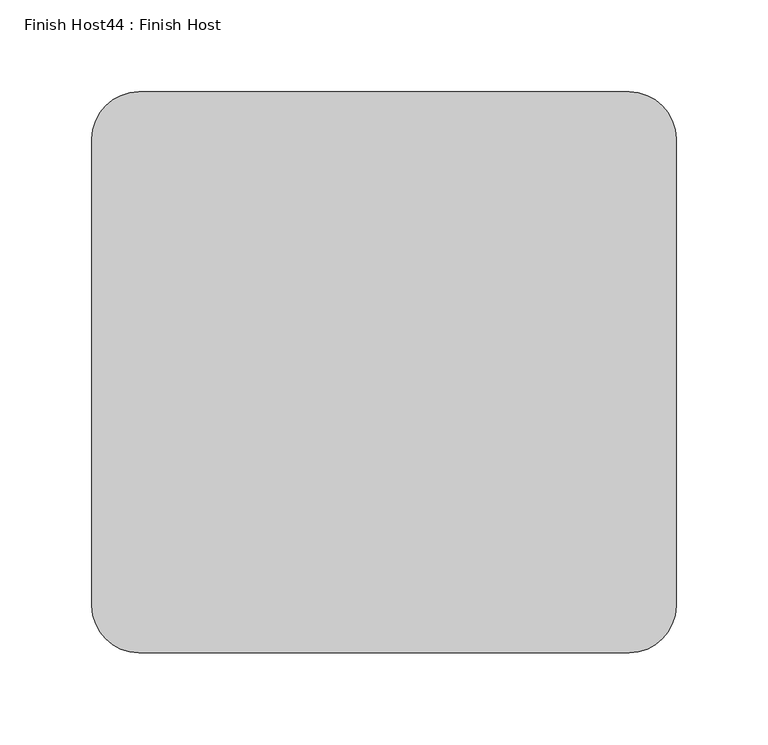
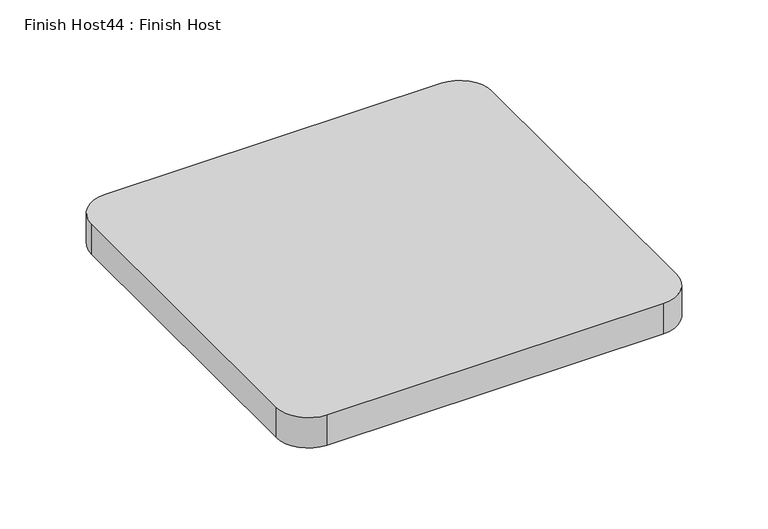
"""IFC4 building model written with IfcOpenShell, lengths in millimetres: proxy geometry, Finish Host44 : Finish Host."""

from ifc_helpers import new_model, si_unit, point, frame_2d, origin, origin_with_axes, place, context, project, spatial, polyline, circle_curve, trimmed, segment, composite_curve, outline, extrude, source, transform, mapped, element, save


def finish_host44_finish_host_5728698f(model_context):
    return source(origin(), model_context, "Body", "SweptSolid", [
        extrude(outline(composite_curve([segment(polyline([(-16287.7939795, 14061.2419385), (-16287.7939795, 14315.2419385)]), True, "CONTINUOUS"), segment(trimmed(circle_curve(frame_2d((-16262.3939795, 14315.2419385)), 25.4), [point((-16287.7939795, 14315.2419385))], [point((-16262.3939795, 14340.6419385))], False, "CARTESIAN"), True, "CONTINUOUS"), segment(polyline([(-16262.3939795, 14340.6419385), (-15995.6939795, 14340.6419385)]), True, "CONTINUOUS"), segment(trimmed(circle_curve(frame_2d((-15995.6939795, 14315.2419385)), 25.4), [point((-15995.6939795, 14340.6419385))], [point((-15970.2939795, 14315.2419385))], False, "CARTESIAN"), True, "CONTINUOUS"), segment(polyline([(-15970.2939795, 14315.2419385), (-15970.2939795, 14061.2419385)]), True, "CONTINUOUS"), segment(trimmed(circle_curve(frame_2d((-15995.6939795, 14061.2419385)), 25.4), [point((-15970.2939795, 14061.2419385))], [point((-15995.6939795, 14035.8419385))], False, "CARTESIAN"), True, "CONTINUOUS"), segment(polyline([(-15995.6939795, 14035.8419385), (-16262.3939795, 14035.8419385)]), True, "CONTINUOUS"), segment(trimmed(circle_curve(frame_2d((-16262.3939795, 14061.2419385)), 25.4), [point((-16262.3939795, 14035.8419385))], [point((-16287.7939795, 14061.2419385))], False, "CARTESIAN"), True, "CONTINUOUS")], self_intersect=False)), origin_with_axes(), (0.0, 0.0, 1.0), 25.4),
    ])


if __name__ == "__main__":
    model = new_model("IFC4")
    model_context = context("Model", 3, world=origin())
    ifc_project = project(units=[si_unit("LENGTHUNIT", "METRE", prefix="MILLI")], contexts=[model_context])
    site = spatial("IfcSite", under=ifc_project)
    building = spatial("IfcBuilding", under=site)
    placement = place(None, origin())
    finish_host44_finish_host_shape = finish_host44_finish_host_5728698f(model_context)
    element("IfcBuildingElementProxy", 1, Name="Finish Host44 : Finish Host", ObjectType="Finish Host44 : Finish Host", at=placement, inside=building, context=model_context, shape_type="MappedRepresentation", body=[
        mapped(finish_host44_finish_host_shape, transform((0.0, 0.0, 0.0), x_axis=(1.0, 0.0, 0.0), y_axis=(0.0, 1.0, 0.0), z_axis=(0.0, 0.0, 1.0))),
    ])
    save(model, "model.ifc")

# Revit data of these elements
# Type "Finish Host44 : Finish Host"
#   Countertop Material = none
# Element 1 (IfcBuildingElementProxy, "Finish Host44 : Finish Host")
#   Materials on its faces: "Thread - Teknion - Silver"
# Materials
#   "Thread - Teknion - Silver": class "Fabric", colour RGB 115 115 117, transparency 0, Model = "F206", Manufacturer = "Teknion Studio", URL = "http://www.teknion.com/", Description = "Fantasme Full Wool", Cost = 0
